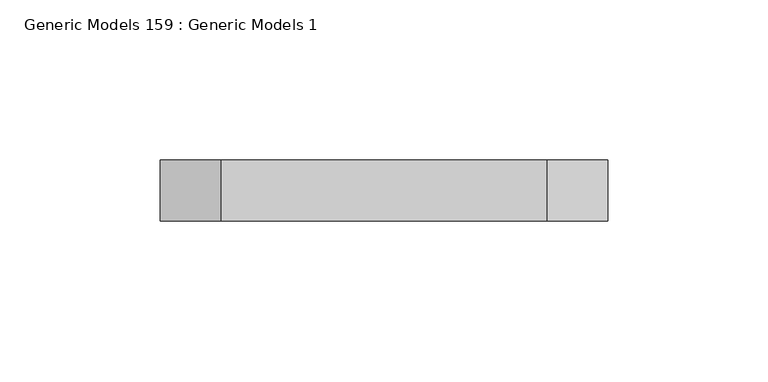
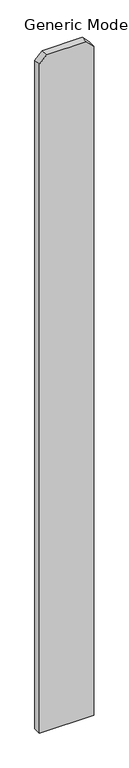
"""IFC4 building model written with IfcOpenShell, lengths in millimetres: proxy geometry, Generic Models 159 : Generic Models 1."""

from ifc_helpers import new_model, si_unit, frame, origin, place, context, project, spatial, polyline, outline, extrude, source, transform, mapped, element, save


def generic_models_159_generic_models_1_27e70c3d(model_context):
    return source(origin(), model_context, "Body", "SweptSolid", [
        extrude(outline(polyline([(76.2, 54227.4125), (1885.95, 54227.4125), (1905.0, 54208.3625), (1905.0, 54106.7625), (1885.95, 54087.7125), (76.2, 54087.7125), (76.2, 54227.4125)])), frame((0.0, 547.6875, 0.0), z_axis=(0.0, 1.0, 0.0), x_axis=(0.0, 0.0, 1.0)), (0.0, 0.0, 1.0), 19.05),
    ])


if __name__ == "__main__":
    model = new_model("IFC4")
    model_context = context("Model", 3, world=origin())
    ifc_project = project(units=[si_unit("LENGTHUNIT", "METRE", prefix="MILLI")], contexts=[model_context])
    site = spatial("IfcSite", under=ifc_project)
    building = spatial("IfcBuilding", under=site)
    placement = place(None, origin())
    generic_models_159_generic_models_1_shape = generic_models_159_generic_models_1_27e70c3d(model_context)
    element("IfcBuildingElementProxy", 1, Name="Generic Models 159 : Generic Models 1", ObjectType="Generic Models 159 : Generic Models 1", at=placement, inside=building, context=model_context, shape_type="MappedRepresentation", body=[
        mapped(generic_models_159_generic_models_1_shape, transform((0.0, 0.0, 0.0), x_axis=(1.0, 0.0, 0.0), y_axis=(0.0, 1.0, 0.0), z_axis=(0.0, 0.0, 1.0))),
    ])
    save(model, "model.ifc")

# Revit data of these elements
# Element 1 (IfcBuildingElementProxy, "Generic Models 159 : Generic Models 1")
#   Materials on its faces: "VERTICAL 1X6 CEDAR PLANKS W/ CLEAR WOOD SEALER"
# Materials
#   "VERTICAL 1X6 CEDAR PLANKS W/ CLEAR WOOD SEALER": class "Wood", colour RGB 234 198 147, transparency 0, Description = "Pinus Echinata", Cost = 0
